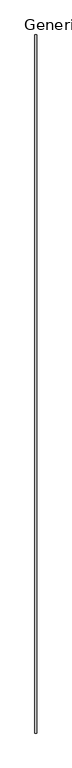
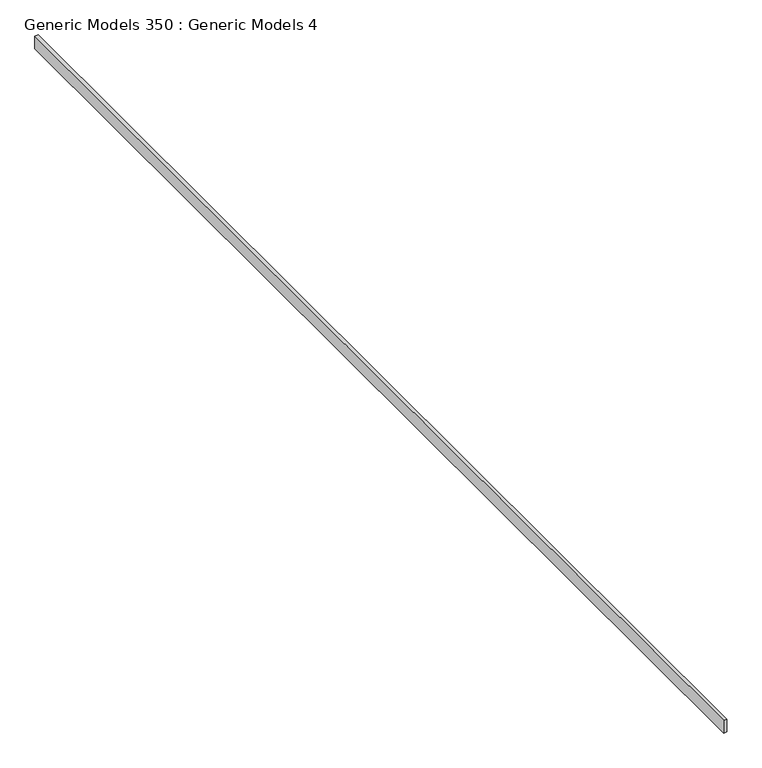
"""IFC4 building model written with IfcOpenShell, lengths in millimetres: proxy geometry, Generic Models 350 : Generic Models 4."""

from ifc_helpers import new_model, si_unit, frame, origin, place, context, project, spatial, polyline, outline, extrude, source, transform, mapped, element, save


def generic_models_350_generic_models_4_0254af19(model_context):
    return source(origin(), model_context, "Body", "SweptSolid", [
        extrude(outline(polyline([(-6421.3539395, -6864.9230338), (-6439.0736296, -6864.9230338), (-6439.0736296, -464.1230338), (-6421.3539395, -464.1230338), (-6421.3539395, -6864.9230338)])), frame((0.0, 0.0, 126802.896), z_axis=(0.0, 0.0, 1.0), x_axis=(1.0, 0.0, 0.0)), (0.0, 0.0, 1.0), 73.7057335),
    ])


if __name__ == "__main__":
    model = new_model("IFC4")
    model_context = context("Model", 3, world=origin())
    ifc_project = project(units=[si_unit("LENGTHUNIT", "METRE", prefix="MILLI")], contexts=[model_context])
    site = spatial("IfcSite", under=ifc_project)
    building = spatial("IfcBuilding", under=site)
    placement = place(None, origin())
    generic_models_350_generic_models_4_shape = generic_models_350_generic_models_4_0254af19(model_context)
    element("IfcBuildingElementProxy", 1, Name="Generic Models 350 : Generic Models 4", ObjectType="Generic Models 350 : Generic Models 4", at=placement, inside=building, context=model_context, shape_type="MappedRepresentation", body=[
        mapped(generic_models_350_generic_models_4_shape, transform((0.0, 0.0, 0.0), x_axis=(1.0, 0.0, 0.0), y_axis=(0.0, 1.0, 0.0), z_axis=(0.0, 0.0, 1.0))),
    ])
    save(model, "model.ifc")

# Revit data of these elements
# Element 1 (IfcBuildingElementProxy, "Generic Models 350 : Generic Models 4")
#   Materials on its faces: "_WOOD FLOORING (SPEC T.B.D.)"
# Materials
#   "_WOOD FLOORING (SPEC T.B.D.)": class "Generic", colour RGB 177 130 114, transparency 0, Cost = 0
